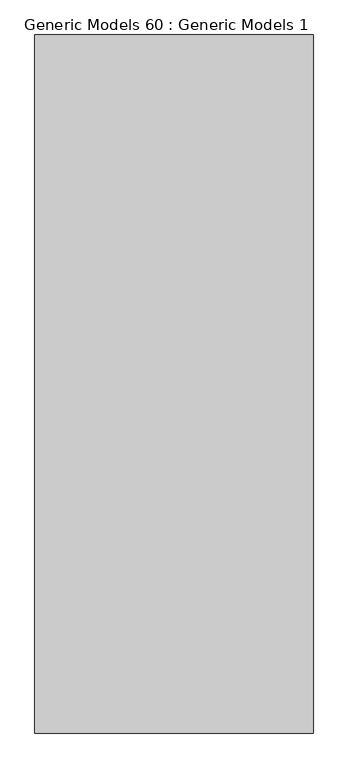
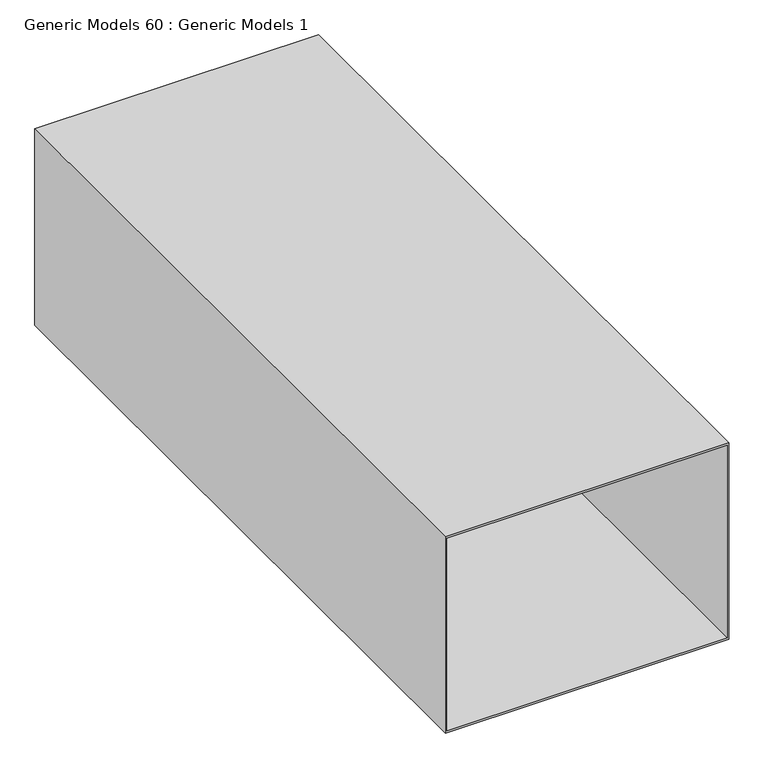
"""IFC4 building model written with IfcOpenShell, lengths in millimetres: proxy geometry, Generic Models 60 : Generic Models 1."""

from ifc_helpers import new_model, si_unit, frame, origin, place, context, project, spatial, polyline, outline, extrude, source, transform, mapped, element, save


def generic_models_60_generic_models_1_d31512ee(model_context):
    return source(origin(), model_context, "Body", "SweptSolid", [
        extrude(outline(polyline([(2028.825, 50664.9319345), (2028.825, 51151.5547769), (2384.425, 51151.5547769), (2384.425, 50664.9319345), (2028.825, 50664.9319345)]), holes=[polyline([(2381.25, 51148.3797769), (2032.0, 51148.3797769), (2032.0, 50668.1069345), (2381.25, 50668.1069345), (2381.25, 51148.3797769)])]), frame((0.0, 0.0, 0.0), z_axis=(0.0, 1.0, 0.0), x_axis=(0.0, 0.0, 1.0)), (0.0, 0.0, 1.0), 1219.2),
    ])


if __name__ == "__main__":
    model = new_model("IFC4")
    model_context = context("Model", 3, world=origin())
    ifc_project = project(units=[si_unit("LENGTHUNIT", "METRE", prefix="MILLI")], contexts=[model_context])
    site = spatial("IfcSite", under=ifc_project)
    building = spatial("IfcBuilding", under=site)
    placement = place(None, origin())
    generic_models_60_generic_models_1_shape = generic_models_60_generic_models_1_d31512ee(model_context)
    element("IfcBuildingElementProxy", 1, Name="Generic Models 60 : Generic Models 1", ObjectType="Generic Models 60 : Generic Models 1", at=placement, inside=building, context=model_context, shape_type="MappedRepresentation", body=[
        mapped(generic_models_60_generic_models_1_shape, transform((0.0, 0.0, 0.0), x_axis=(1.0, 0.0, 0.0), y_axis=(0.0, 1.0, 0.0), z_axis=(0.0, 0.0, 1.0))),
    ])
    save(model, "model.ifc")

# Revit data of these elements
# Element 1 (IfcBuildingElementProxy, "Generic Models 60 : Generic Models 1")
#   Materials on its faces: "EXISTING DUCT"
# Materials
#   "EXISTING DUCT": class "Generic", colour RGB 120 120 120, transparency 0, Cost = 0
